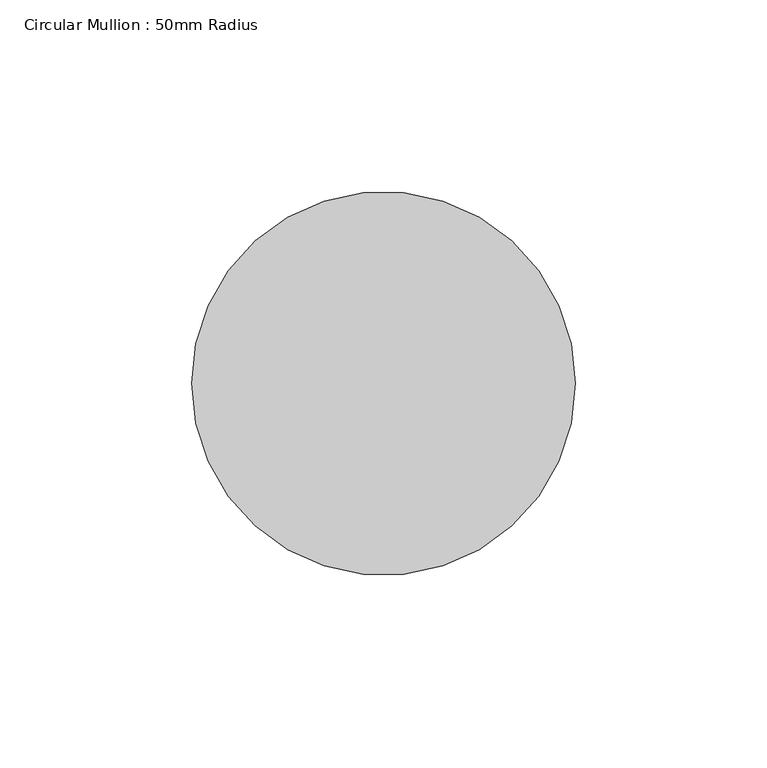
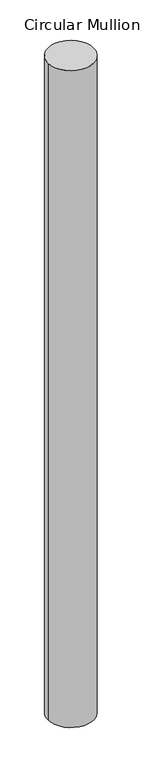
"""IFC4 building model written with IfcOpenShell, lengths in millimetres: member geometry, Circular Mullion : 50mm Radius."""

from ifc_helpers import new_model, si_unit, point, frame, origin, origin_2d, place, context, project, spatial, circle_curve, trimmed, segment, composite_curve, outline, extrude, source, transform, mapped, element, save


def circular_mullion_50mm_radius_fab7c51c(model_context):
    return source(origin(), model_context, "Body", "SweptSolid", [
        extrude(outline(composite_curve([segment(trimmed(circle_curve(origin_2d(), 50.0), [point((50.0, 0.0))], [point((-50.0, 0.0))], False, "CARTESIAN"), True, "CONTINUOUS"), segment(trimmed(circle_curve(origin_2d(), 50.0), [point((-50.0, 0.0))], [point((50.0, 0.0))], False, "CARTESIAN"), True, "CONTINUOUS")], self_intersect=False)), frame((0.0, 0.0, -1516.8695329), z_axis=(0.0, 0.0, 1.0), x_axis=(1.0, 0.0, 0.0)), (0.0, 0.0, 1.0), 1516.8695329),
    ])


if __name__ == "__main__":
    model = new_model("IFC4")
    model_context = context("Model", 3, world=origin())
    ifc_project = project(units=[si_unit("LENGTHUNIT", "METRE", prefix="MILLI")], contexts=[model_context])
    site = spatial("IfcSite", under=ifc_project)
    building = spatial("IfcBuilding", under=site)
    placement = place(None, origin())
    circular_mullion_50mm_radius_shape = circular_mullion_50mm_radius_fab7c51c(model_context)
    element("IfcMember", 1, ObjectType="Circular Mullion : 50mm Radius", at=placement, inside=building, context=model_context, shape_type="MappedRepresentation", body=[
        mapped(circular_mullion_50mm_radius_shape, transform((0.0, 0.0, 0.0), x_axis=(1.0, 0.0, 0.0), y_axis=(0.0, 1.0, 0.0), z_axis=(0.0, 0.0, 1.0))),
    ])
    save(model, "model.ifc")

# Revit data of these elements
# Type "Circular Mullion : 50mm Radius"
#   built-in parameter 1007350 = 0.164042 (stored number, unit not read)
# Element 1 (IfcMember, "Circular Mullion : 50mm Radius")
#   Materials on its faces: "Aluminium"
# Materials
#   "Aluminium": class "Metal", colour RGB 247 247 247, transparency 0, Description = "Aluminium 6061", Cost = 0
